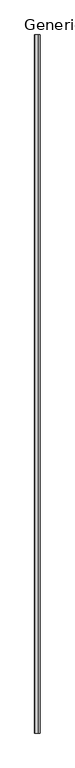
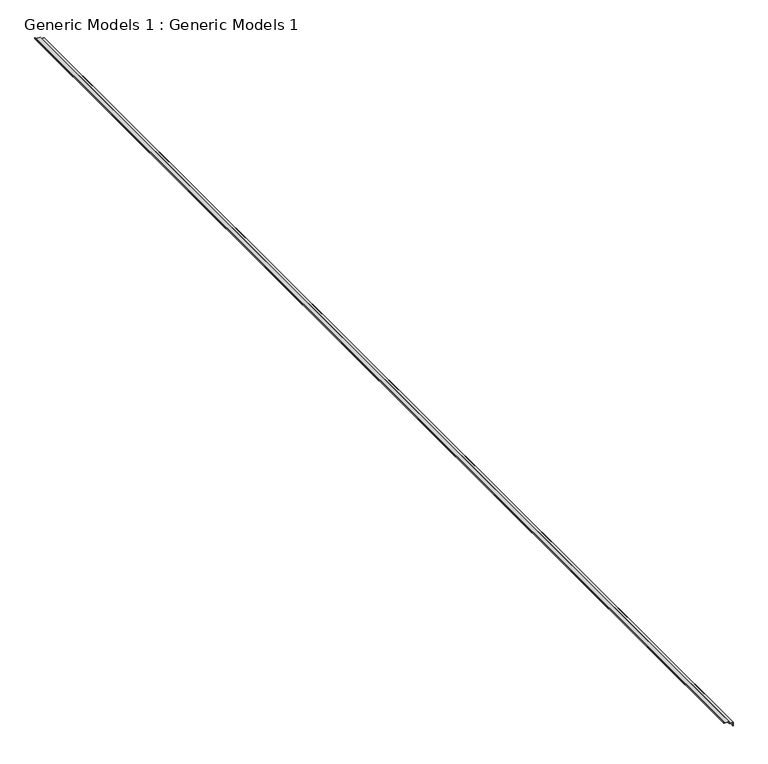
"""IFC4 building model written with IfcOpenShell, lengths in millimetres: proxy geometry, Generic Models 1 : Generic Models 1."""

from ifc_helpers import new_model, si_unit, frame, origin, place, context, project, spatial, polyline, outline, extrude, source, transform, mapped, element, save


def generic_models_1_generic_models_1_639715c1(model_context):
    return source(origin(), model_context, "Body", "SweptSolid", [
        extrude(outline(polyline([(266403.9811486, 32099.1399105), (266403.9811486, 32165.3220884), (266378.5811486, 32165.3220884), (266378.5811486, 32213.5326935), (266331.370214, 32213.5326935), (266331.370214, 32215.1201935), (266380.1686486, 32215.1201935), (266380.1686486, 32166.9095884), (266405.5686486, 32166.9095884), (266405.5686486, 32100.7274105), (266417.2431924, 32100.7274105), (266417.2431924, 32099.1399105), (266403.9811486, 32099.1399105)])), frame((0.0, 25672.1156612, 0.0), z_axis=(0.0, 1.0, 0.0), x_axis=(0.0, 0.0, 1.0)), (0.0, 0.0, 1.0), 15155.545),
    ])


if __name__ == "__main__":
    model = new_model("IFC4")
    model_context = context("Model", 3, world=origin())
    ifc_project = project(units=[si_unit("LENGTHUNIT", "METRE", prefix="MILLI")], contexts=[model_context])
    site = spatial("IfcSite", under=ifc_project)
    building = spatial("IfcBuilding", under=site)
    placement = place(None, origin())
    generic_models_1_generic_models_1_shape = generic_models_1_generic_models_1_639715c1(model_context)
    element("IfcBuildingElementProxy", 1, Name="Generic Models 1 : Generic Models 1", ObjectType="Generic Models 1 : Generic Models 1", at=placement, inside=building, context=model_context, shape_type="MappedRepresentation", body=[
        mapped(generic_models_1_generic_models_1_shape, transform((0.0, 0.0, 0.0), x_axis=(1.0, 0.0, 0.0), y_axis=(0.0, 1.0, 0.0), z_axis=(0.0, 0.0, 1.0))),
    ])
    save(model, "model.ifc")

# Revit data of these elements
# Element 1 (IfcBuildingElementProxy, "Generic Models 1 : Generic Models 1")
#   Materials on its faces: "GALV. BRAKE METAL - (COLOR: DARK BRONZE)"
# Materials
#   "GALV. BRAKE METAL - (COLOR: DARK BRONZE)": class "Generic", colour RGB 72 52 47, transparency 0, Cost = 0
